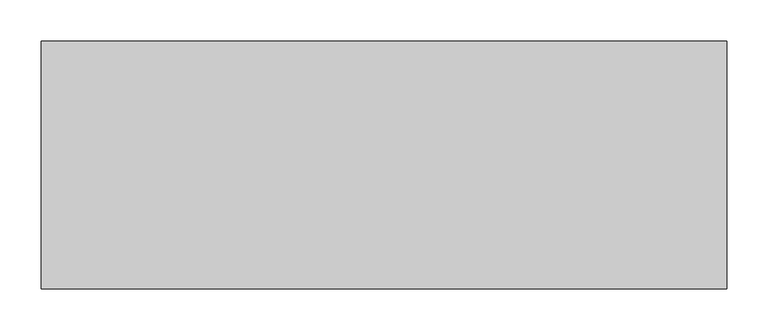
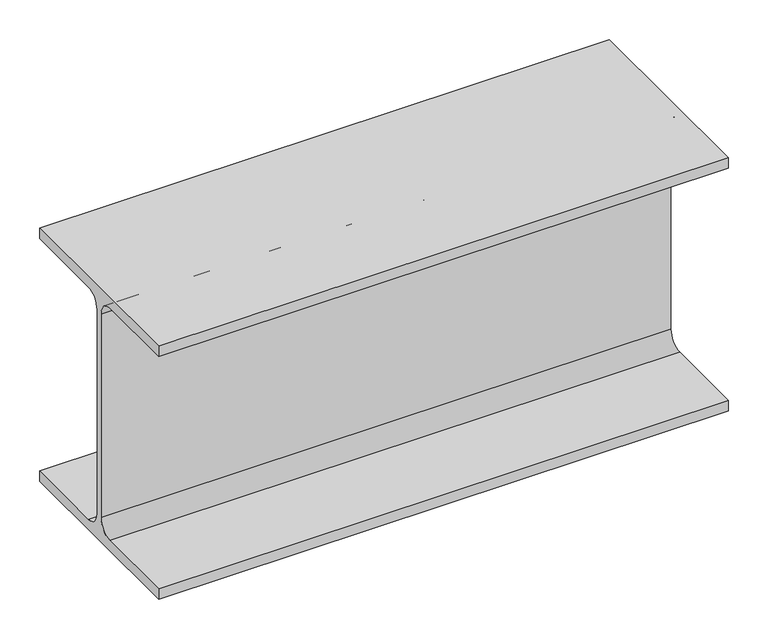
"""IFC4 building model written with IfcOpenShell, lengths in millimetres: beam geometry, 0912_Steel Framing_H-KSD3502 : H_SB_ASB_H-390x300x10x16."""

from ifc_helpers import new_model, si_unit, point, frame, frame_2d, origin, place, context, project, spatial, polyline, circle_curve, trimmed, segment, composite_curve, outline, extrude, source, transform, mapped, element, save


def beam_b61b1237(model_context):
    return source(origin(), model_context, "Body", "SweptSolid", [
        extrude(outline(composite_curve([segment(polyline([(150.0, -179.0), (150.0, -195.0), (-150.0, -195.0), (-150.0, -179.0), (-27.0, -179.0)]), True, "CONTINUOUS"), segment(trimmed(circle_curve(frame_2d((-27.0, -157.0)), 22.0), [point((-27.0, -179.0))], [point((-5.0, -157.0))], True, "CARTESIAN"), True, "CONTINUOUS"), segment(polyline([(-5.0, -157.0), (-5.0, 157.0)]), True, "CONTINUOUS"), segment(trimmed(circle_curve(frame_2d((-27.0, 157.0)), 22.0), [point((-5.0, 157.0))], [point((-27.0, 179.0))], True, "CARTESIAN"), True, "CONTINUOUS"), segment(polyline([(-27.0, 179.0), (-150.0, 179.0), (-150.0, 195.0), (150.0, 195.0), (150.0, 179.0), (27.0, 179.0)]), True, "CONTINUOUS"), segment(trimmed(circle_curve(frame_2d((27.0, 157.0)), 22.0), [point((27.0, 179.0))], [point((5.0, 157.0))], True, "CARTESIAN"), True, "CONTINUOUS"), segment(polyline([(5.0, 157.0), (5.0, -157.0)]), True, "CONTINUOUS"), segment(trimmed(circle_curve(frame_2d((27.0, -157.0)), 22.0), [point((5.0, -157.0))], [point((27.0, -179.0))], True, "CARTESIAN"), True, "CONTINUOUS"), segment(polyline([(27.0, -179.0), (150.0, -179.0)]), True, "CONTINUOUS")], self_intersect=False)), frame((-415.0, 0.0, 0.0), z_axis=(1.0, 0.0, 0.0), x_axis=(0.0, 1.0, 0.0)), (0.0, 0.0, 1.0), 830.0),
    ])


if __name__ == "__main__":
    model = new_model("IFC4")
    model_context = context("Model", 3, world=origin())
    ifc_project = project(units=[si_unit("LENGTHUNIT", "METRE", prefix="MILLI")], contexts=[model_context])
    site = spatial("IfcSite", under=ifc_project)
    building = spatial("IfcBuilding", under=site)
    placement = place(None, origin())
    beam_shape = beam_b61b1237(model_context)
    element("IfcBeam", 1, ObjectType="0912_Steel Framing_H-KSD3502 : H_SB_ASB_H-390x300x10x16", at=placement, inside=building, context=model_context, shape_type="MappedRepresentation", body=[
        mapped(beam_shape, transform((0.0, 0.0, 0.0), x_axis=(1.0, 0.0, 0.0), y_axis=(0.0, 1.0, 0.0), z_axis=(0.0, 0.0, 1.0))),
    ])
    save(model, "model.ifc")

# Revit data of these elements
# Type "0912_Steel Framing_H-KSD3502 : H_SB_ASB_H-390x300x10x16"
#   H_WM Code_1 = "S01AA001-00001 | Main Steel Structure Fabrication Work | Shelter/Building | Heavy Steel - Standard (Weight≥90KG/M) | Material: (   )"
#   H_WM Code_2 = "S03AA027-00001 | Main Steel Structure Erection Work | Shelter/Building | Heavy Steel (Weight≥90KG/M) | Material: (   )"
#   H_WM Code_3 = "S01AA010-00001 | Main Steel Structure Fabrication Work | Shelter/Building | Steel Painting/Coating | for Non-Fireproofed Steel Surface, Surface Preparation, Primer, Second & Final Coat | Material: (   )"
#   H_Q'ty Cal Type Tag = "SB-Q2"
#   Width = 30.0 cm
#   Web Thickness = 1.0 cm
#   Web Fillet = 2.2 cm
#   Warping Constant = 2520000.0 cm⁶
#   W = 0
#   Torsional Moment of Inertia = 94.3867 cm⁴
#   Section Area = 136.0 cm²
#   Plastic Modulus weak axis = 733.0 cm³
#   Plastic Modulus strong axis = 2190.0 cm³
#   Perimeter = 1.92 m²/m
#   Nominal Weight = 107.00 kgf/m
#   Moment of Inertia weak axis = 7210.00 cm⁴
#   Moment of Inertia strong axis = 38700.00 cm⁴
#   Height = 39.0 cm
#   Flange Thickness = 1.6 cm
#   Elastic Modulus weak axis = 481.0 cm³
#   Elastic Modulus strong axis = 1980.0 cm³
#   Centroid Vertical = 19.5 cm
#   Centroid Horizontal = 15.0 cm
#   Ix = 387000000
#   Length [instance default] = 1.5240 m
#   Zx = 2190000
#   b = 0.3000 m
#   h = 0.3900 m
#   r = 0.0220 m
#   s = 0.0100 m
#   t = 0.0160 m
#   A = 0.0136 m²
#   Structural Material [instance default] = Steel, 45-345
#   Assembly Code = ""
# Element 1 (IfcBeam, "0912_Steel Framing_H-KSD3502 : H_SB_ASB_H-390x300x10x16")
#   Structural Material = none
# Materials
#   "Steel, 45-345": class "Metal", colour RGB 189 187 185, transparency 0, Description = "Steel 345 MPa", Cost = 0
